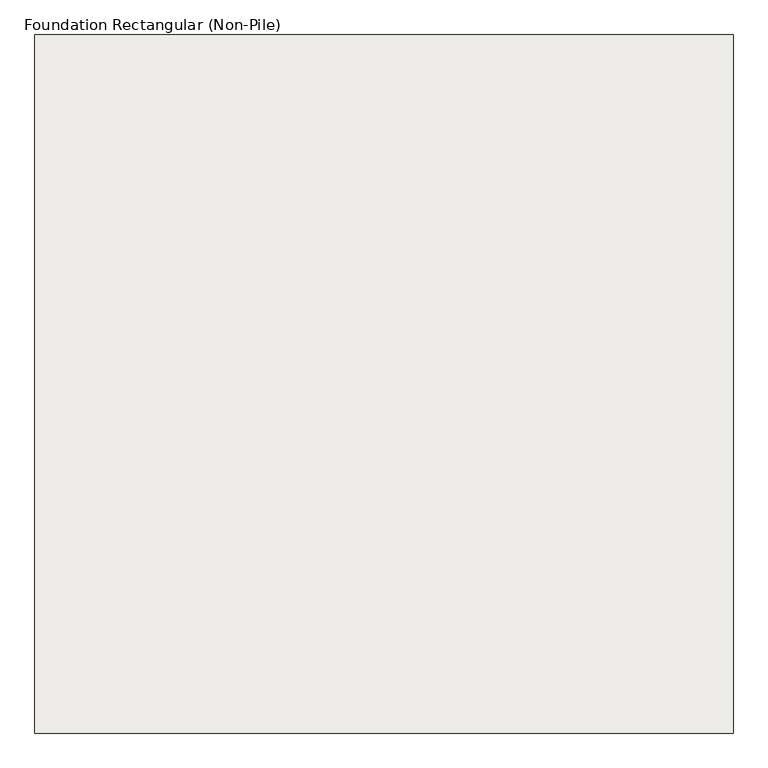
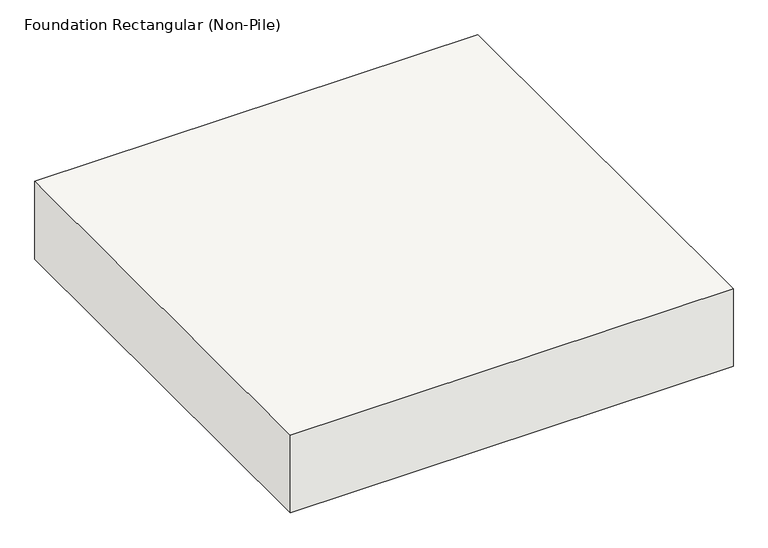
"""IFC4 building model written with IfcOpenShell, lengths in millimetres: slab geometry, Foundation Rectangular (Non-Pile) : H_SF_AR S18_Ret Fdn_F1 2700x2700x500."""

from ifc_helpers import new_model, si_unit, frame, origin, place, context, project, spatial, polyline, outline, extrude, source, transform, mapped, element, save


def foundation_rectangular_non_pile_db20e422(model_context):
    return source(origin(), model_context, "Body", "SweptSolid", [
        extrude(outline(polyline([(1350.0, 1350.0), (1350.0, -1350.0), (-1350.0, -1350.0), (-1350.0, 1350.0), (1350.0, 1350.0)])), frame((0.0, 0.0, -500.0), z_axis=(0.0, 0.0, 1.0), x_axis=(1.0, 0.0, 0.0)), (0.0, 0.0, 1.0), 500.0),
    ])


if __name__ == "__main__":
    model = new_model("IFC4")
    model_context = context("Model", 3, world=origin())
    ifc_project = project(units=[si_unit("LENGTHUNIT", "METRE", prefix="MILLI")], contexts=[model_context])
    site = spatial("IfcSite", under=ifc_project)
    building = spatial("IfcBuilding", under=site)
    placement = place(None, origin())
    foundation_rectangular_non_pile_shape = foundation_rectangular_non_pile_db20e422(model_context)
    element("IfcSlab", 1, ObjectType="Foundation Rectangular (Non-Pile) : H_SF_AR S18_Ret Fdn_F1 2700x2700x500", at=placement, inside=building, context=model_context, shape_type="MappedRepresentation", body=[
        mapped(foundation_rectangular_non_pile_shape, transform((0.0, 0.0, 0.0), x_axis=(1.0, 0.0, 0.0), y_axis=(0.0, 1.0, 0.0), z_axis=(0.0, 0.0, 1.0))),
    ])
    save(model, "model.ifc")

# Revit data of these elements
# Type "Foundation Rectangular (Non-Pile) : H_SF_AR S18_Ret Fdn_F1 2700x2700x500"
#   Type Comments = "UG"
#   Type Mark = "F1"
#   Top bar = "D25@300"
#   Description = "UG Shallow Foundation"
#   Bottom bar = "D20@300"
#   H_Rebar Ratio = 0.12
#   Width = 2700 mm
#   Length = 2700 mm
#   Foundation Thickness = 500 mm
#   Structural Material [instance default] = none
#   Assembly Code = ""
# Element 1 (IfcSlab, "Foundation Rectangular (Non-Pile) : H_SF_AR S18_Ret Fdn_F1 2700x2700x500")
#   Materials on its faces: "00_Concrete_Reinf. Conc."
# Materials
#   "00_Concrete_Reinf. Conc.": class "Concrete", colour RGB 176 176 176, transparency 0, Description = "Reinf. Conc.", Cost = 0, Image = Concrete.Cast-In-Place.Flat.Polished.Grey.jpg
